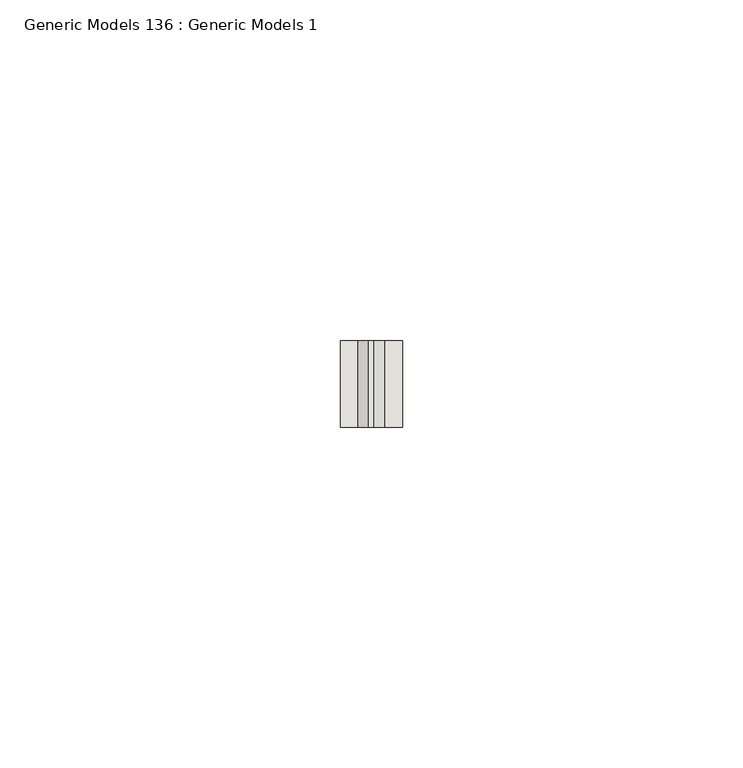
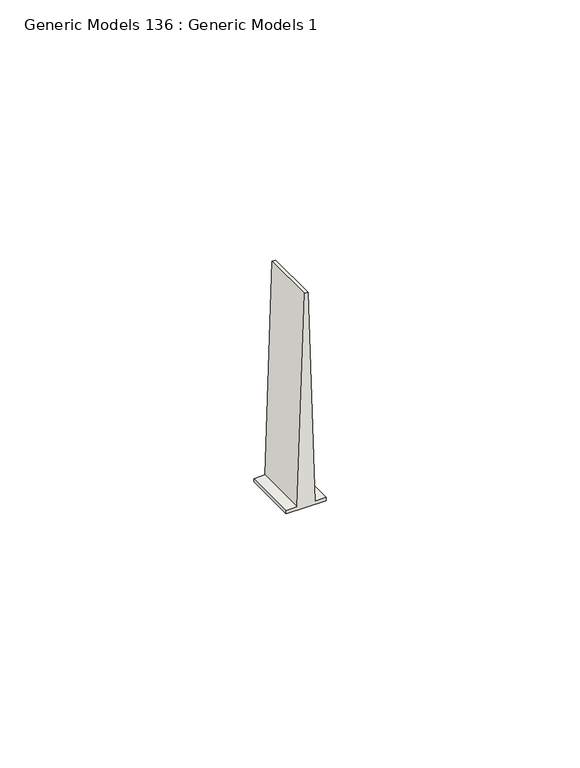
"""IFC4 building model written with IfcOpenShell, lengths in millimetres: wall geometry, Generic Models 136 : Generic Models 1."""

from ifc_helpers import new_model, si_unit, frame, origin, place, context, project, spatial, polyline, outline, extrude, source, transform, mapped, element, save


def generic_models_136_generic_models_1_822dc4f7(model_context):
    return source(origin(), model_context, "Body", "SweptSolid", [
        extrude(outline(polyline([(2455.06875, 50952.6159), (2455.06875, 50961.7091), (2455.8625, 50961.7091), (2455.8625, 50959.1592364), (2506.6625, 50957.5618473), (2506.6625, 50956.7631527), (2455.8625, 50955.1657636), (2455.8625, 50952.6159), (2455.06875, 50952.6159)])), frame((0.0, 565.15, 0.0), z_axis=(0.0, 1.0, 0.0), x_axis=(0.0, 0.0, 1.0)), (0.0, 0.0, 1.0), 12.7),
    ])


if __name__ == "__main__":
    model = new_model("IFC4")
    model_context = context("Model", 3, world=origin())
    ifc_project = project(units=[si_unit("LENGTHUNIT", "METRE", prefix="MILLI")], contexts=[model_context])
    site = spatial("IfcSite", under=ifc_project)
    building = spatial("IfcBuilding", under=site)
    placement = place(None, origin())
    generic_models_136_generic_models_1_shape = generic_models_136_generic_models_1_822dc4f7(model_context)
    element("IfcWall", 1, ObjectType="Generic Models 136 : Generic Models 1", at=placement, inside=building, context=model_context, shape_type="MappedRepresentation", body=[
        mapped(generic_models_136_generic_models_1_shape, transform((0.0, 0.0, 0.0), x_axis=(1.0, 0.0, 0.0), y_axis=(0.0, 1.0, 0.0), z_axis=(0.0, 0.0, 1.0))),
    ])
    save(model, "model.ifc")

# Revit data of these elements
# Element 1 (IfcWall, "Generic Models 136 : Generic Models 1")
#   Materials on its faces: "METAL RUNNER CHANNEL; FASTEN @ 24\" O.C."
# Materials
#   "METAL RUNNER CHANNEL; FASTEN @ 24\" O.C.": class "Unassigned", colour RGB 210 209 208, transparency 0, Keynote = "M05121300.02", Cost = 0
